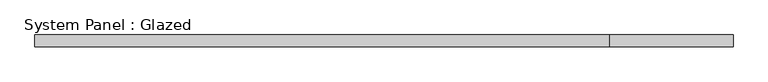
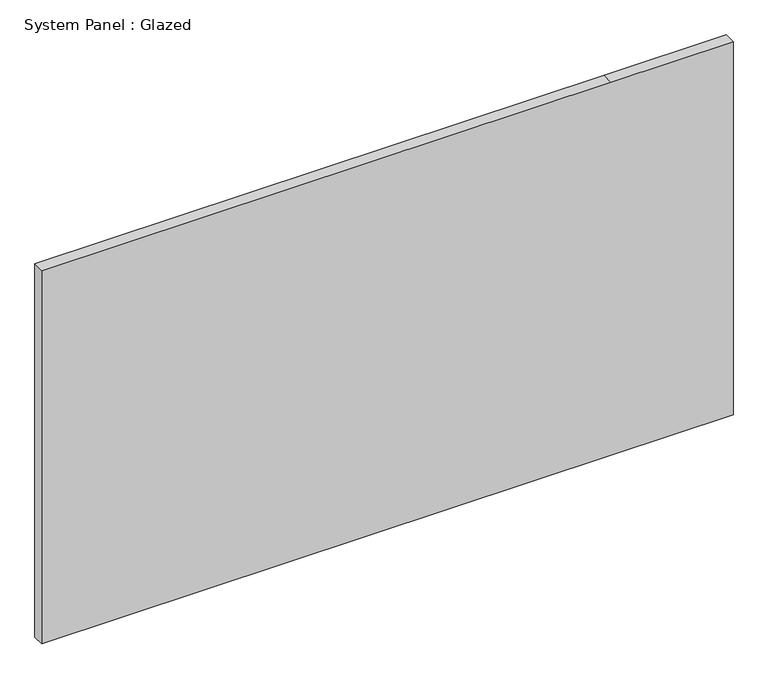
"""IFC4 building model written with IfcOpenShell, lengths in millimetres: plate geometry, System Panel : Glazed."""

from ifc_helpers import new_model, si_unit, frame, origin, place, context, project, spatial, polyline, outline, extrude, source, transform, mapped, element, save


def system_panel_glazed_62768381(model_context):
    return source(origin(), model_context, "Body", "SweptSolid", [
        extrude(outline(polyline([(0.0, -756.44375), (0.0, 488.95), (0.0, 756.44375), (863.6, 756.44375), (863.6, 488.95), (863.6, -756.44375), (0.0, -756.44375)])), frame((0.0, -44.45, 0.0), z_axis=(0.0, 1.0, 0.0), x_axis=(0.0, 0.0, 1.0)), (0.0, 0.0, 1.0), 25.4),
    ])


if __name__ == "__main__":
    model = new_model("IFC4")
    model_context = context("Model", 3, world=origin())
    ifc_project = project(units=[si_unit("LENGTHUNIT", "METRE", prefix="MILLI")], contexts=[model_context])
    site = spatial("IfcSite", under=ifc_project)
    building = spatial("IfcBuilding", under=site)
    placement = place(None, origin())
    system_panel_glazed_shape = system_panel_glazed_62768381(model_context)
    element("IfcPlate", 1, ObjectType="System Panel : Glazed", at=placement, inside=building, context=model_context, shape_type="MappedRepresentation", body=[
        mapped(system_panel_glazed_shape, transform((0.0, 0.0, 0.0), x_axis=(1.0, 0.0, 0.0), y_axis=(0.0, 1.0, 0.0), z_axis=(0.0, 0.0, 1.0))),
    ])
    save(model, "model.ifc")

# Revit data of these elements
# Element 1 (IfcPlate, "System Panel : Glazed")
#   Materials on its faces: "Glass"
# Materials
#   "Glass": class "Glass", colour RGB 0 128 192, transparency 0.75, Cost = 0
